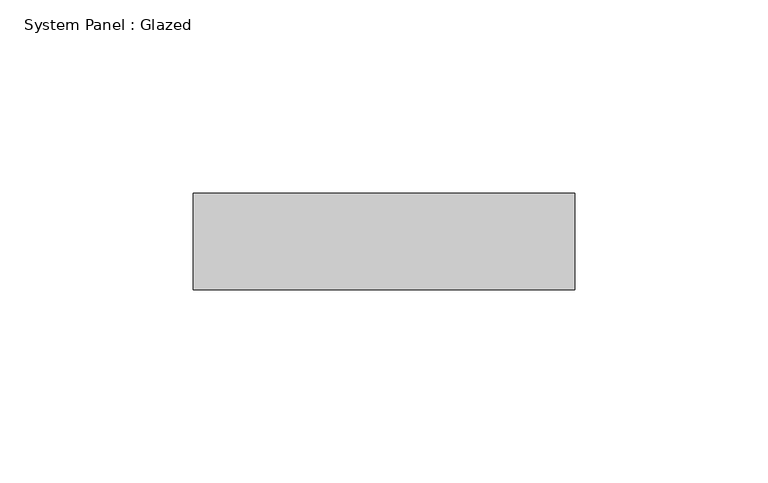
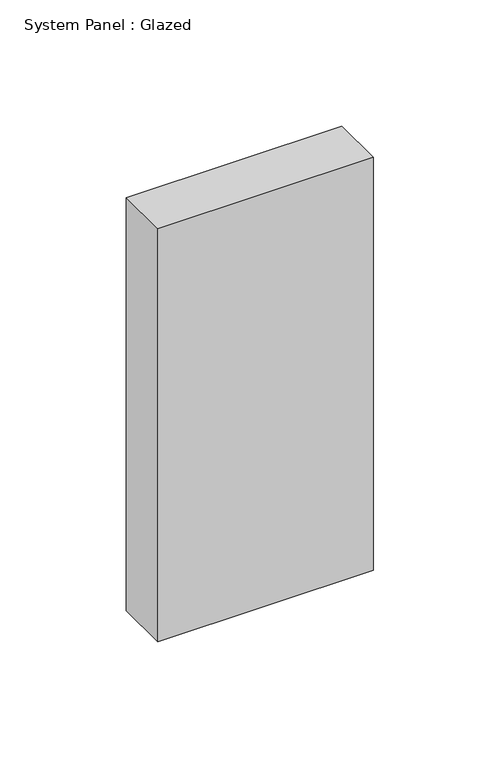
"""IFC4 building model written with IfcOpenShell, lengths in millimetres: plate geometry, System Panel : Glazed."""

from ifc_helpers import new_model, si_unit, origin, origin_with_axes, place, context, project, spatial, polyline, outline, extrude, source, transform, mapped, element, save


def system_panel_glazed_3dd544b4(model_context):
    return source(origin(), model_context, "Body", "SweptSolid", [
        extrude(outline(polyline([(49.4357818, 24.5), (-49.4357818, 24.5), (-49.4357818, 49.5), (49.4357818, 49.5), (49.4357818, 24.5)])), origin_with_axes(), (0.0, 0.0, 1.0), 200.0),
    ])


if __name__ == "__main__":
    model = new_model("IFC4")
    model_context = context("Model", 3, world=origin())
    ifc_project = project(units=[si_unit("LENGTHUNIT", "METRE", prefix="MILLI")], contexts=[model_context])
    site = spatial("IfcSite", under=ifc_project)
    building = spatial("IfcBuilding", under=site)
    placement = place(None, origin())
    system_panel_glazed_shape = system_panel_glazed_3dd544b4(model_context)
    element("IfcPlate", 1, ObjectType="System Panel : Glazed", at=placement, inside=building, context=model_context, shape_type="MappedRepresentation", body=[
        mapped(system_panel_glazed_shape, transform((0.0, 0.0, 0.0), x_axis=(1.0, 0.0, 0.0), y_axis=(0.0, 1.0, 0.0), z_axis=(0.0, 0.0, 1.0))),
    ])
    save(model, "model.ifc")

# Revit data of these elements
# Element 1 (IfcPlate, "System Panel : Glazed")
#   Materials on its faces: "Glass"
# Materials
#   "Glass": class "Glass", colour RGB 218 227 224, transparency 0.85, Description = "Soda Lime Glass", Cost = 0
